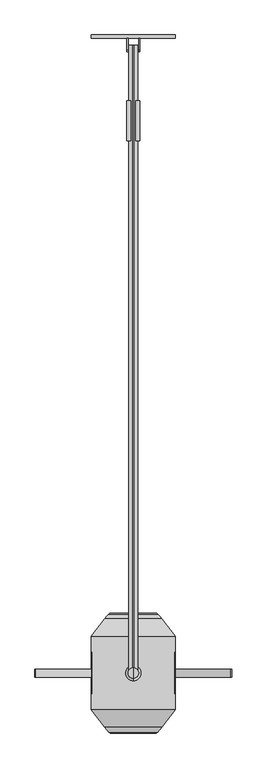
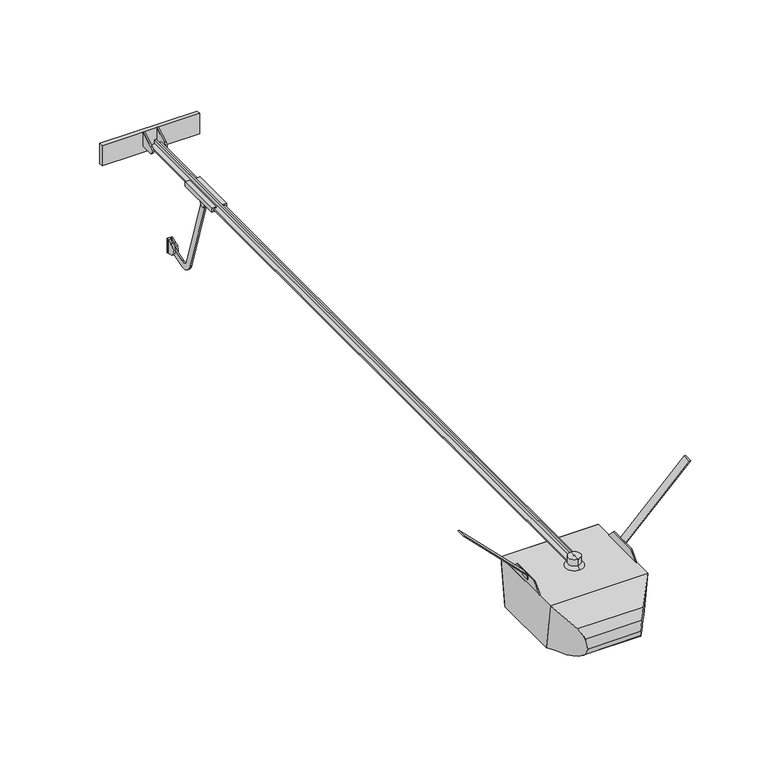
"""IFC4 building model written with IfcOpenShell, lengths in millimetres: proxy geometry, DoorOpener_Garage_Liftmaster_Residential-Standard : DoorOpener_Garage_Liftmaster_Residential-Standard."""

from ifc_helpers import new_model, si_unit, point, frame, frame_2d, origin, place, context, project, spatial, polyline, circle_curve, ellipse_curve, trimmed, segment, composite_curve, outline, extrude, source, transform, mapped, element, save
from ifc_brep_helpers import plane_surface, cylinder_surface, revolved_surface, advanced_brep


def specialty_equipment_f89a715d(model_context):
    return source(origin(), model_context, "Body", "SolidModel", [
        advanced_brep(
        [(-203.2, 149.6475517, -508.0003876), (203.2, 149.6475517, -508.0003876), (203.2, 177.8000484, -304.8), (-203.2, 177.8000484, -304.8), (138.0453476, 261.2609425, -380.4314301), (-138.0453476, 261.2609425, -380.4314301), (-118.4954842, 284.259248, -417.8810822), (118.4954842, 284.259248, -417.8810822), (-110.84057, 289.2573619, -461.4672022), (110.84057, 289.2573619, -461.4672022), (-116.7901976, 276.5450386, -491.3073174), (116.7901976, 276.5450386, -491.3073174), (-130.1422035, 255.1783195, -506.5798347), (130.1422035, 255.1783195, -506.5798347), (-170.8715769, 195.6710506, -512.2392761), (170.8715769, 195.6710506, -512.2392761)],
        [
            (0, 1),
            (1, 2),
            (2, 3),
            (3, 0),
            (2, 4, ellipse_curve(frame((725.3174618, -724.5630466, -1384.4430479), z_axis=(-0.8191520442889955, -0.5681495809146607, 0.0787145605568323), x_axis=(-0.5735764363510407, 0.8114016915146515, -0.11241604276082225)), 1717.7336421, 1407.0850245)),
            (4, 5),
            (5, 3, ellipse_curve(frame((-725.3174618, -724.5630466, -1384.4430479), z_axis=(0.8191520442889911, -0.5681495809146667, 0.07871456055683229), x_axis=(-0.573576436351047, -0.8114016915146469, 0.11241604276082202)), 1717.7336421, 1407.0850245)),
            (6, 5, ellipse_curve(frame((-176.0372598, 197.4858414, -445.3831284), z_axis=(0.8191520442889911, -0.5681495809146667, 0.07871456055683229), x_axis=(-0.573576436351047, -0.8114016915146469, 0.11241604276082202)), 111.1239307, 91.027395)),
            (4, 7, ellipse_curve(frame((176.0372598, 197.4858414, -445.3831284), z_axis=(-0.8191520442889955, -0.5681495809146607, 0.0787145605568323), x_axis=(-0.5735764363510407, 0.8114016915146515, -0.11241604276082225)), 111.1239307, 91.027395)),
            (7, 6),
            (8, 6, ellipse_curve(frame((-190.88231, 175.0994001, -452.4783085), z_axis=(0.8191520442889911, -0.5681495809146667, 0.07871456055683229), x_axis=(-0.573576436351047, -0.8114016915146469, 0.11241604276082202)), 139.7924992, 114.5113115)),
            (7, 9, ellipse_curve(frame((190.88231, 175.0994001, -452.4783085), z_axis=(-0.8191520442889955, -0.5681495809146607, 0.0787145605568323), x_axis=(-0.5735764363510407, 0.8114016915146515, -0.11241604276082225)), 139.7924992, 114.5113115)),
            (9, 8),
            (10, 8, ellipse_curve(frame((-146.4314203, 238.4966097, -457.470258), z_axis=(0.8191520442889911, -0.5681495809146667, 0.07871456055683229), x_axis=(-0.573576436351047, -0.8114016915146469, 0.11241604276082202)), 62.1592423, 50.9178704)),
            (9, 11, ellipse_curve(frame((146.4314203, 238.4966097, -457.470258), z_axis=(-0.8191520442889955, -0.5681495809146607, 0.0787145605568323), x_axis=(-0.5735764363510407, 0.8114016915146515, -0.11241604276082225)), 62.1592423, 50.9178704)),
            (11, 10),
            (12, 10, ellipse_curve(frame((-151.3050469, 232.2406655, -451.9067495), z_axis=(0.8191520442889911, -0.5681495809146667, 0.07871456055683229), x_axis=(-0.573576436351047, -0.8114016915146469, 0.11241604276082202)), 72.3795001, 59.2898155)),
            (11, 13, ellipse_curve(frame((151.3050469, 232.2406655, -451.9067495), z_axis=(-0.8191520442889955, -0.5681495809146607, 0.0787145605568323), x_axis=(-0.5735764363510407, 0.8114016915146515, -0.11241604276082225)), 72.3795001, 59.2898155)),
            (13, 12),
            (14, 12, ellipse_curve(frame((-165.9618007, 216.3547308, -414.0418022), z_axis=(0.8191520442889911, -0.5681495809146667, 0.07871456055683229), x_axis=(-0.573576436351047, -0.8114016915146469, 0.11241604276082202)), 122.507382, 100.3521724)),
            (13, 15, ellipse_curve(frame((165.9618007, 216.3547308, -414.0418022), z_axis=(-0.8191520442889955, -0.5681495809146607, 0.0787145605568323), x_axis=(-0.5735764363510407, 0.8114016915146515, -0.11241604276082225)), 122.507382, 100.3521724)),
            (15, 14),
            (0, 14, ellipse_curve(frame((-180.6608006, 154.4314578, -708.0276372), z_axis=(-0.8191520442889911, 0.5681495809146667, -0.07871456055683229), x_axis=(0.573576436351047, 0.8114016915146469, -0.11241604276082202)), 244.2580098, 200.0844481)),
            (15, 1, ellipse_curve(frame((180.6608006, 154.4314578, -708.0276372), z_axis=(0.8191520442889955, 0.5681495809146607, -0.0787145605568323), x_axis=(0.5735764363510407, -0.8114016915146515, 0.11241604276082225)), 244.2580098, 200.0844481)),
        ],
        [
            plane_surface(frame((-203.2, 149.6475517, -508.0003876), z_axis=(0.0, -0.9905385662791439, 0.13723464837153254), x_axis=(1.0, 0.0, 0.0))),
            cylinder_surface(frame((203.2, -724.5630466, -1384.4430479), z_axis=(-1.0, 0.0, 0.0), x_axis=(0.0, 1.0, 0.0)), 1407.0850245),
            cylinder_surface(frame((203.2, 197.4858414, -445.3831284), z_axis=(-1.0, 0.0, 0.0), x_axis=(0.0, 1.0, 0.0)), 91.027395),
            cylinder_surface(frame((203.2, 175.0994001, -452.4783085), z_axis=(-1.0, 0.0, 0.0), x_axis=(0.0, 1.0, 0.0)), 114.5113115),
            cylinder_surface(frame((203.2, 238.4966097, -457.470258), z_axis=(-1.0, 0.0, 0.0), x_axis=(0.0, 1.0, 0.0)), 50.9178704),
            cylinder_surface(frame((203.2, 232.2406655, -451.9067495), z_axis=(-1.0, 0.0, 0.0), x_axis=(0.0, 1.0, 0.0)), 59.2898155),
            cylinder_surface(frame((203.2, 216.3547308, -414.0418022), z_axis=(-1.0, 0.0, 0.0), x_axis=(0.0, 1.0, 0.0)), 100.3521724),
            revolved_surface(polyline([(320.7614394112816, 354.5159059, -708.0276372), (-320.7614394112831, 354.5159059, -708.0276372)]), (203.2, 154.4314578, -708.0276372), (1.0, 0.0, 0.0)),
            plane_surface(frame((-74.2567818, 321.5979485, -608.7511868), z_axis=(-0.8191520442889911, 0.5681495809146667, -0.07871456055683229), x_axis=(0.0, 0.13723464837153243, 0.9905385662791438))),
            plane_surface(frame((74.2567818, 369.5271494, -262.8055925), z_axis=(0.8191520442889955, 0.5681495809146607, -0.0787145605568323), x_axis=(0.0, -0.1372346483715328, -0.9905385662791438))),
        ],
        [
            (0, [[1, 2, 3, 4]]),
            (1, [[-3, 5, 6, 7]]),
            (2, [[8, -6, 9, 10]]),
            (3, [[11, -10, 12, 13]]),
            (4, [[14, -13, 15, 16]]),
            (5, [[17, -16, 18, 19]]),
            (6, [[20, -19, 21, 22]]),
            (7, [[-1, 23, -22, 24]]),
            (8, [[-4, -7, -8, -11, -14, -17, -20, -23]]),
            (9, [[-2, -24, -21, -18, -15, -12, -9, -5]]),
        ],
    ),
        extrude(outline(polyline([(177.8000484, -304.8), (149.6475517, -508.0003876), (-149.6475517, -508.0003876), (-177.8000484, -304.8), (177.8000484, -304.8)])), frame((-203.2, 0.0, 0.0), z_axis=(1.0, 0.0, 0.0), x_axis=(0.0, 1.0, 0.0)), (0.0, 0.0, 1.0), 406.4),
        advanced_brep(
        [(-203.2, -149.6475517, -508.0003876), (203.2, -149.6475517, -508.0003876), (170.8715769, -195.6710506, -512.2392761), (-170.8715769, -195.6710506, -512.2392761), (-130.1422035, -255.1783195, -506.5798347), (130.1422035, -255.1783195, -506.5798347), (-116.7901976, -276.5450386, -491.3073174), (116.7901976, -276.5450386, -491.3073174), (-110.84057, -289.2573619, -461.4672022), (110.84057, -289.2573619, -461.4672022), (-118.4954842, -284.259248, -417.8810822), (118.4954842, -284.259248, -417.8810822), (-138.0453476, -261.2609425, -380.4314301), (138.0453476, -261.2609425, -380.4314301), (203.2, -177.8000484, -304.8), (-203.2, -177.8000484, -304.8)],
        [
            (0, 1),
            (1, 2, ellipse_curve(frame((180.6608006, -154.4314578, -708.0276372), z_axis=(0.8191520442889902, -0.568149580914668, -0.07871456055683303), x_axis=(0.5735764363510483, 0.8114016915146459, 0.11241604276082269)), 244.2580098, 200.0844481)),
            (2, 3),
            (3, 0, ellipse_curve(frame((-180.6608006, -154.4314578, -708.0276372), z_axis=(-0.8191520442889942, -0.5681495809146623, -0.07871456055683314), x_axis=(0.5735764363510426, -0.8114016915146501, -0.11241604276082295)), 244.2580098, 200.0844481)),
            (4, 3, ellipse_curve(frame((-165.9618007, -216.3547308, -414.0418022), z_axis=(0.8191520442889942, 0.5681495809146623, 0.07871456055683314), x_axis=(-0.5735764363510426, 0.8114016915146501, 0.11241604276082295)), 122.507382, 100.3521724)),
            (2, 5, ellipse_curve(frame((165.9618007, -216.3547308, -414.0418022), z_axis=(-0.8191520442889902, 0.568149580914668, 0.07871456055683303), x_axis=(-0.5735764363510483, -0.8114016915146459, -0.11241604276082269)), 122.507382, 100.3521724)),
            (5, 4),
            (6, 4, ellipse_curve(frame((-151.3050469, -232.2406655, -451.9067495), z_axis=(0.8191520442889942, 0.5681495809146623, 0.07871456055683314), x_axis=(-0.5735764363510426, 0.8114016915146501, 0.11241604276082295)), 72.3795001, 59.2898155)),
            (5, 7, ellipse_curve(frame((151.3050469, -232.2406655, -451.9067495), z_axis=(-0.8191520442889902, 0.568149580914668, 0.07871456055683303), x_axis=(-0.5735764363510483, -0.8114016915146459, -0.11241604276082269)), 72.3795001, 59.2898155)),
            (7, 6),
            (8, 6, ellipse_curve(frame((-146.4314203, -238.4966097, -457.470258), z_axis=(0.8191520442889942, 0.5681495809146623, 0.07871456055683314), x_axis=(-0.5735764363510426, 0.8114016915146501, 0.11241604276082295)), 62.1592423, 50.9178704)),
            (7, 9, ellipse_curve(frame((146.4314203, -238.4966097, -457.470258), z_axis=(-0.8191520442889902, 0.568149580914668, 0.07871456055683303), x_axis=(-0.5735764363510483, -0.8114016915146459, -0.11241604276082269)), 62.1592423, 50.9178704)),
            (9, 8),
            (10, 8, ellipse_curve(frame((-190.88231, -175.0994001, -452.4783085), z_axis=(0.8191520442889942, 0.5681495809146623, 0.07871456055683314), x_axis=(-0.5735764363510426, 0.8114016915146501, 0.11241604276082295)), 139.7924992, 114.5113115)),
            (9, 11, ellipse_curve(frame((190.88231, -175.0994001, -452.4783085), z_axis=(-0.8191520442889902, 0.568149580914668, 0.07871456055683303), x_axis=(-0.5735764363510483, -0.8114016915146459, -0.11241604276082269)), 139.7924992, 114.5113115)),
            (11, 10),
            (12, 10, ellipse_curve(frame((-176.0372598, -197.4858414, -445.3831284), z_axis=(0.8191520442889942, 0.5681495809146623, 0.07871456055683314), x_axis=(-0.5735764363510426, 0.8114016915146501, 0.11241604276082295)), 111.1239307, 91.027395)),
            (11, 13, ellipse_curve(frame((176.0372598, -197.4858414, -445.3831284), z_axis=(-0.8191520442889902, 0.568149580914668, 0.07871456055683303), x_axis=(-0.5735764363510483, -0.8114016915146459, -0.11241604276082269)), 111.1239307, 91.027395)),
            (13, 12),
            (14, 15),
            (15, 12, ellipse_curve(frame((-725.3174618, 724.5630466, -1384.4430479), z_axis=(0.8191520442889942, 0.5681495809146623, 0.07871456055683314), x_axis=(-0.5735764363510426, 0.8114016915146501, 0.11241604276082295)), 1717.7336421, 1407.0850245)),
            (13, 14, ellipse_curve(frame((725.3174618, 724.5630466, -1384.4430479), z_axis=(-0.8191520442889902, 0.568149580914668, 0.07871456055683303), x_axis=(-0.5735764363510483, -0.8114016915146459, -0.11241604276082269)), 1717.7336421, 1407.0850245)),
            (0, 15),
            (14, 1),
        ],
        [
            revolved_surface(polyline([(320.7614394112834, -354.5159059, -708.0276372), (-320.76143941128197, -354.5159059, -708.0276372)]), (203.2, -154.4314578, -708.0276372), (1.0, 0.0, 0.0)),
            cylinder_surface(frame((203.2, -216.3547308, -414.0418022), z_axis=(-1.0, 0.0, 0.0), x_axis=(0.0, -1.0, 0.0)), 100.3521724),
            cylinder_surface(frame((203.2, -232.2406655, -451.9067495), z_axis=(-1.0, 0.0, 0.0), x_axis=(0.0, -1.0, 0.0)), 59.2898155),
            cylinder_surface(frame((203.2, -238.4966097, -457.470258), z_axis=(-1.0, 0.0, 0.0), x_axis=(0.0, -1.0, 0.0)), 50.9178704),
            cylinder_surface(frame((203.2, -175.0994001, -452.4783085), z_axis=(-1.0, 0.0, 0.0), x_axis=(0.0, -1.0, 0.0)), 114.5113115),
            cylinder_surface(frame((203.2, -197.4858414, -445.3831284), z_axis=(-1.0, 0.0, 0.0), x_axis=(0.0, -1.0, 0.0)), 91.027395),
            cylinder_surface(frame((203.2, 724.5630466, -1384.4430479), z_axis=(-1.0, 0.0, 0.0), x_axis=(0.0, -1.0, 0.0)), 1407.0850245),
            plane_surface(frame((-203.2, -177.8000484, -304.8), z_axis=(0.0, 0.9905385662791436, 0.13723464837153496), x_axis=(1.0, 0.0, 0.0))),
            plane_surface(frame((-203.2, -142.6760316, -558.3197467), z_axis=(-0.8191520442889942, -0.5681495809146623, -0.07871456055683314), x_axis=(0.0, -0.13723464837153365, 0.9905385662791437))),
            plane_surface(frame((203.2, -196.7053127, -168.3447132), z_axis=(0.81915204428899, -0.5681495809146679, -0.07871456055683301), x_axis=(0.0, 0.13723464837153368, -0.9905385662791437))),
        ],
        [
            (0, [[1, 2, 3, 4]]),
            (1, [[5, -3, 6, 7]]),
            (2, [[8, -7, 9, 10]]),
            (3, [[11, -10, 12, 13]]),
            (4, [[14, -13, 15, 16]]),
            (5, [[17, -16, 18, 19]]),
            (6, [[20, 21, -19, 22]]),
            (7, [[-1, 23, -20, 24]]),
            (8, [[-4, -5, -8, -11, -14, -17, -21, -23]]),
            (9, [[-2, -24, -22, -18, -15, -12, -9, -6]]),
        ],
    ),
        extrude(outline(polyline([(-285.75, -203.2), (-266.7, -203.2), (0.0, -469.9), (0.0, -474.3901281), (-268.0151281, -206.375), (-285.75, -206.375), (-285.75, -203.2)])), frame((0.0, -19.05, 0.0), z_axis=(0.0, 1.0, 0.0), x_axis=(0.0, 0.0, 1.0)), (0.0, 0.0, 1.0), 38.1),
        extrude(outline(polyline([(-285.75, 203.2), (-285.75, 206.375), (-268.0151281, 206.375), (0.0, 474.3901281), (0.0, 469.9), (-266.7, 203.2), (-285.75, 203.2)])), frame((0.0, -19.05, 0.0), z_axis=(0.0, 1.0, 0.0), x_axis=(0.0, 0.0, 1.0)), (0.0, 0.0, 1.0), 38.1),
        advanced_brep(
        [(31.75, 2758.489219, -277.7618368), (31.75, 2566.8381944, -277.7618368), (31.75, 2566.8381944, -296.0931426), (31.75, 2758.489219, -296.0931426), (-31.75, 2758.489219, -296.0931426), (-31.75, 2566.8381944, -296.0931426), (-31.75, 2566.8381944, -277.7618368), (-31.75, 2758.489219, -277.7618368), (9.525, 2758.489219, -296.0931426), (9.525, 2758.489219, -304.8), (-9.525, 2758.489219, -304.8), (-9.525, 2758.489219, -296.0931426), (-12.7, 2758.489219, -277.7618368), (-12.7, 2758.489219, -282.575), (-22.225, 2758.489219, -282.575), (-22.225, 2758.489219, -288.925), (22.225, 2758.489219, -288.925), (22.225, 2758.489219, -282.575), (12.7, 2758.489219, -282.575), (12.7, 2758.489219, -277.7618368), (12.7, 2566.8381944, -277.7618368), (-12.7, 2566.8381944, -277.7618368), (12.7, 2566.8381944, -282.575), (22.225, 2566.8381944, -282.575), (22.225, 2566.8381944, -288.925), (-22.225, 2566.8381944, -288.925), (-22.225, 2566.8381944, -282.575), (-12.7, 2566.8381944, -282.575), (-9.525, 2611.2881944, -296.0931426), (9.525, 2611.2881944, -296.0931426), (-9.525, 2616.3151009, -304.8), (9.525, 2616.3151009, -304.8), (-9.525, 2647.8709399, -304.8), (9.525, 2647.8709399, -304.8), (-9.525, 2658.7300795, -334.6352407), (9.525, 2658.7300795, -334.6352407), (-9.525, 2684.1300795, -334.6352407), (9.525, 2684.1300795, -334.6352407), (-9.525, 2694.989219, -304.8), (9.525, 2694.989219, -304.8)],
        [
            (0, 1),
            (1, 2),
            (2, 3),
            (3, 0),
            (4, 5),
            (5, 6),
            (6, 7),
            (7, 4),
            (3, 8),
            (8, 9),
            (9, 10),
            (10, 11),
            (11, 4),
            (7, 12),
            (12, 13),
            (13, 14),
            (14, 15),
            (15, 16),
            (16, 17),
            (17, 18),
            (18, 19),
            (19, 0),
            (19, 20),
            (20, 1),
            (6, 21),
            (21, 12),
            (5, 2),
            (20, 22),
            (22, 23),
            (23, 24),
            (24, 25),
            (25, 26),
            (26, 27),
            (27, 21),
            (11, 28),
            (28, 29),
            (29, 8),
            (28, 30),
            (30, 31),
            (31, 29),
            (30, 32),
            (32, 33),
            (33, 31),
            (32, 34),
            (34, 35),
            (35, 33),
            (34, 36, circle_curve(frame((-9.525, 2671.4300795, -330.0128187), z_axis=(1.0, 0.0, 0.0), x_axis=(0.0, 1.0, 0.0)), 13.5150577)),
            (36, 37),
            (37, 35, circle_curve(frame((9.525, 2671.4300795, -330.0128187), z_axis=(-1.0, 0.0, 0.0), x_axis=(0.0, 1.0, 0.0)), 13.5150577)),
            (36, 38),
            (38, 39),
            (39, 37),
            (9, 39),
            (38, 10),
            (13, 27),
            (26, 14),
            (25, 15),
            (24, 16),
            (23, 17),
            (22, 18),
        ],
        [
            plane_surface(frame((31.75, 2758.489219, -277.7618368), z_axis=(1.0, 0.0, 0.0), x_axis=(0.0, 0.0, 1.0))),
            plane_surface(frame((-31.75, 2758.489219, -277.7618368), z_axis=(-1.0, 0.0, 0.0), x_axis=(0.0, 0.0, -1.0))),
            plane_surface(frame((31.75, 2758.489219, -304.8), z_axis=(0.0, 1.0, 0.0), x_axis=(-1.0, 0.0, 0.0))),
            plane_surface(frame((31.75, 2758.489219, -277.7618368), z_axis=(0.0, 0.0, 1.0), x_axis=(-1.0, 0.0, 0.0))),
            plane_surface(frame((31.75, 2566.8381944, -277.7618368), z_axis=(0.0, -1.0, 0.0), x_axis=(-1.0, 0.0, 0.0))),
            plane_surface(frame((31.75, 2566.8381944, -296.0931426), z_axis=(0.0, 0.0, -1.0), x_axis=(-1.0, 0.0, 0.0))),
            plane_surface(frame((31.75, 2611.2881944, -296.0931426), z_axis=(0.0, -0.8660254037844414, -0.4999999999999954), x_axis=(-1.0, 0.0, 0.0))),
            plane_surface(frame((31.75, 2616.3151009, -304.8), z_axis=(0.0, 0.0, -1.0), x_axis=(-1.0, 0.0, 0.0))),
            plane_surface(frame((31.75, 2647.8709399, -304.8), z_axis=(0.0, -0.9396926207858758, -0.3420201433257583), x_axis=(-1.0, 0.0, 0.0))),
            cylinder_surface(frame((-31.75, 2671.4300795, -330.0128187), z_axis=(1.0, 0.0, 0.0), x_axis=(0.0, 1.0, 0.0)), 13.5150577),
            plane_surface(frame((31.75, 2684.1300795, -334.6352407), z_axis=(0.0, 0.939692620785905, -0.34202014332567826), x_axis=(-1.0, 0.0, 0.0))),
            plane_surface(frame((31.75, 2694.989219, -304.8), z_axis=(0.0, 0.0, -1.0), x_axis=(-1.0, 0.0, 0.0))),
            plane_surface(frame((-12.7, 2529.0462818, -282.575), z_axis=(0.0, 0.0, -1.0), x_axis=(0.0, 1.0, 0.0))),
            plane_surface(frame((-22.225, 2529.0462818, -282.575), z_axis=(1.0, 0.0, 0.0), x_axis=(0.0, 1.0, 0.0))),
            plane_surface(frame((-22.225, 2529.0462818, -288.925), z_axis=(0.0, 0.0, 1.0), x_axis=(0.0, 1.0, 0.0))),
            plane_surface(frame((22.225, 2529.0462818, -288.925), z_axis=(-1.0, 0.0, 0.0), x_axis=(0.0, 1.0, 0.0))),
            plane_surface(frame((22.225, 2529.0462818, -282.575), z_axis=(0.0, 0.0, -1.0), x_axis=(0.0, 1.0, 0.0))),
            plane_surface(frame((12.7, 2529.0462818, -282.575), z_axis=(-1.0, 0.0, 0.0), x_axis=(0.0, 1.0, 0.0))),
            plane_surface(frame((9.525, 2529.0462818, -296.0931426), z_axis=(1.0, 0.0, 0.0), x_axis=(0.0, 1.0, 0.0))),
            plane_surface(frame((-9.525, 2529.0462818, -350.5128419), z_axis=(-1.0, 0.0, 0.0), x_axis=(0.0, 1.0, 0.0))),
            plane_surface(frame((-12.7, 2529.0462818, -274.6526549), z_axis=(1.0, 0.0, 0.0), x_axis=(0.0, 1.0, 0.0))),
        ],
        [
            (0, [[1, 2, 3, 4]]),
            (1, [[5, 6, 7, 8]]),
            (2, [[-4, 9, 10, 11, 12, 13, -8, 14, 15, 16, 17, 18, 19, 20, 21, 22]]),
            (3, [[-1, -22, 23, 24]]),
            (3, [[-7, 25, 26, -14]]),
            (4, [[27, -2, -24, 28, 29, 30, 31, 32, 33, 34, -25, -6]]),
            (5, [[-13, 35, 36, 37, -9, -3, -27, -5]]),
            (6, [[-36, 38, 39, 40]]),
            (7, [[-39, 41, 42, 43]]),
            (8, [[-42, 44, 45, 46]]),
            (9, [[-45, 47, 48, 49]]),
            (10, [[-48, 50, 51, 52]]),
            (11, [[-11, 53, -51, 54]]),
            (12, [[55, -33, 56, -16]]),
            (13, [[-56, -32, 57, -17]]),
            (14, [[-57, -31, 58, -18]]),
            (15, [[-58, -30, 59, -19]]),
            (16, [[-59, -29, 60, -20]]),
            (17, [[-60, -28, -23, -21]]),
            (18, [[-37, -40, -43, -46, -49, -52, -53, -10]]),
            (19, [[-35, -12, -54, -50, -47, -44, -41, -38]]),
            (20, [[-55, -15, -26, -34]]),
        ],
    ),
        advanced_brep(
        [(0.0, 25.4, -263.525), (0.0, -25.4, -263.525), (0.0, 0.0, -263.525), (0.0, 25.4, -292.1), (0.0, -25.4, -292.1), (0.0, 38.1, -304.8), (0.0, -38.1, -304.8), (0.0, 0.0, -304.8)],
        [
            (0, 1, circle_curve(frame((0.0, 0.0, -263.525), z_axis=(0.0, 0.0, 1.0), x_axis=(0.0, -1.0, 0.0)), 25.4)),
            (1, 2),
            (2, 0),
            (1, 0, circle_curve(frame((0.0, 0.0, -263.525), z_axis=(0.0, 0.0, 1.0), x_axis=(0.0, -1.0, 0.0)), 25.4)),
            (3, 4, circle_curve(frame((0.0, 0.0, -292.1), z_axis=(0.0, 0.0, 1.0), x_axis=(0.0, -1.0, 0.0)), 25.4)),
            (4, 1),
            (0, 3),
            (4, 3, circle_curve(frame((0.0, 0.0, -292.1), z_axis=(0.0, 0.0, 1.0), x_axis=(0.0, -1.0, 0.0)), 25.4)),
            (5, 6, circle_curve(frame((0.0, 0.0, -304.8), z_axis=(0.0, 0.0, 1.0), x_axis=(0.0, -1.0, 0.0)), 38.1)),
            (6, 4),
            (3, 5),
            (6, 5, circle_curve(frame((0.0, 0.0, -304.8), z_axis=(0.0, 0.0, 1.0), x_axis=(0.0, -1.0, 0.0)), 38.1)),
            (7, 6),
            (5, 7),
        ],
        [
            plane_surface(frame((0.0, 0.0, -263.525), z_axis=(0.0, 0.0, 1.0), x_axis=(0.0, -1.0, 0.0))),
            cylinder_surface(frame((0.0, 0.0, -248.8162134), z_axis=(0.0, 0.0, -1.0), x_axis=(0.0, -1.0, 0.0)), 25.4),
            revolved_surface(polyline([(0.0, -25.4, -292.1), (0.0, -38.1, -304.8)]), (0.0, 0.0, -248.8162134), (0.0, 0.0, -1.0)),
            plane_surface(frame((0.0, 0.0, -304.8), z_axis=(0.0, 0.0, -1.0), x_axis=(0.0, -1.0, 0.0))),
        ],
        [
            (0, [[1, 2, 3]]),
            (0, [[4, -3, -2]]),
            (1, [[5, 6, -1, 7]]),
            (1, [[8, -7, -4, -6]]),
            (2, [[9, 10, -5, 11]]),
            (2, [[12, -11, -8, -10]]),
            (3, [[13, -9, 14]]),
            (3, [[-14, -12, -13]]),
        ],
    ),
        extrude(outline(polyline([(2924.175, -635.0), (2924.175, -698.5), (2917.825, -696.7985226), (2917.825, -636.7014774), (2924.175, -635.0)])), frame((-9.525, 0.0, 0.0), z_axis=(1.0, 0.0, 0.0), x_axis=(0.0, 1.0, 0.0)), (0.0, 0.0, 1.0), 19.05),
        extrude(outline(composite_curve([segment(polyline([(2924.175, -635.0), (2924.175, -698.5), (2897.2464471, -691.284516)]), True, "CONTINUOUS"), segment(trimmed(circle_curve(frame_2d((2903.8204508, -666.75)), 25.4), [point((2897.2464471, -691.284516))], [point((2897.2464471, -642.215484))], False, "CARTESIAN"), True, "CONTINUOUS"), segment(polyline([(2897.2464471, -642.215484), (2924.175, -635.0)]), True, "CONTINUOUS")], self_intersect=False)), frame((-9.525, 0.0, 0.0), z_axis=(1.0, 0.0, 0.0), x_axis=(0.0, 1.0, 0.0)), (0.0, 0.0, 1.0), 6.35),
        extrude(outline(composite_curve([segment(trimmed(circle_curve(frame_2d((2903.8204508, -666.75)), 12.7), [point((2899.895935, -654.6715822))], [point((2907.7449666, -678.8284178))], False, "CARTESIAN"), True, "CONTINUOUS"), segment(polyline([(2907.7449666, -678.8284178), (2835.2744601, -702.3755127)]), True, "CONTINUOUS"), segment(trimmed(circle_curve(frame_2d((2819.5763968, -654.0618417)), 50.8), [point((2835.2744601, -702.3755127))], [point((2771.2627258, -669.759905))], False, "CARTESIAN"), True, "CONTINUOUS"), segment(polyline([(2771.2627258, -669.759905), (2651.564993, -301.3681634), (2675.7218285, -293.5191318), (2795.4195613, -661.9108734)]), True, "CONTINUOUS"), segment(trimmed(circle_curve(frame_2d((2819.5763968, -654.0618417)), 25.4), [point((2795.4195613, -661.9108734))], [point((2827.4254284, -678.2186772))], True, "CARTESIAN"), True, "CONTINUOUS"), segment(polyline([(2827.4254284, -678.2186772), (2899.895935, -654.6715822)]), True, "CONTINUOUS")], self_intersect=False)), frame((-3.175, 0.0, 0.0), z_axis=(1.0, 0.0, 0.0), x_axis=(0.0, 1.0, 0.0)), (0.0, 0.0, 1.0), 6.35),
        extrude(outline(composite_curve([segment(polyline([(2924.175, -635.0), (2924.175, -698.5), (2897.2464471, -691.284516)]), True, "CONTINUOUS"), segment(trimmed(circle_curve(frame_2d((2903.8204508, -666.75)), 25.4), [point((2897.2464471, -691.284516))], [point((2897.2464471, -642.215484))], False, "CARTESIAN"), True, "CONTINUOUS"), segment(polyline([(2897.2464471, -642.215484), (2924.175, -635.0)]), True, "CONTINUOUS")], self_intersect=False)), frame((3.175, 0.0, 0.0), z_axis=(1.0, 0.0, 0.0), x_axis=(0.0, 1.0, 0.0)), (0.0, 0.0, 1.0), 6.35),
        extrude(outline(polyline([(-282.575, -3.175), (-282.575, -22.225), (-288.925, -22.225), (-288.925, 22.225), (-282.575, 22.225), (-282.575, 3.175), (-263.525, 3.175), (-263.525, -3.175), (-282.575, -3.175)])), frame((0.0, 0.0, 0.0), z_axis=(0.0, 1.0, 0.0), x_axis=(0.0, 0.0, 1.0)), (0.0, 0.0, 1.0), 3025.775),
        extrude(outline(composite_curve([segment(polyline([(3060.7, -304.8), (3005.7074265, -304.8)]), True, "CONTINUOUS"), segment(trimmed(circle_curve(frame_2d((3014.8728406, -288.925)), 18.3308604), [point((3005.7074265, -304.8))], [point((3005.7074265, -273.05))], False, "CARTESIAN"), True, "CONTINUOUS"), segment(polyline([(3005.7074265, -273.05), (3060.7, -241.3000969), (3060.7, -304.8)]), True, "CONTINUOUS")], self_intersect=False)), frame((-31.75, 0.0, 0.0), z_axis=(1.0, 0.0, 0.0), x_axis=(0.0, 1.0, 0.0)), (0.0, 0.0, 1.0), 6.35),
        extrude(outline(composite_curve([segment(polyline([(3060.7, -304.8), (3005.7074265, -304.8)]), True, "CONTINUOUS"), segment(trimmed(circle_curve(frame_2d((3014.8728406, -288.925)), 18.3308604), [point((3005.7074265, -304.8))], [point((3005.7074265, -273.05))], False, "CARTESIAN"), True, "CONTINUOUS"), segment(polyline([(3005.7074265, -273.05), (3060.7, -241.3000969), (3060.7, -304.8)]), True, "CONTINUOUS")], self_intersect=False)), frame((25.4, 0.0, 0.0), z_axis=(1.0, 0.0, 0.0), x_axis=(0.0, 1.0, 0.0)), (0.0, 0.0, 1.0), 6.35),
        extrude(outline(polyline([(-203.2, 3076.575), (203.2, 3076.575), (203.2, 3060.7), (-203.2, 3060.7), (-203.2, 3076.575)])), frame((0.0, 0.0, -330.2), z_axis=(0.0, 0.0, 1.0), x_axis=(1.0, 0.0, 0.0)), (0.0, 0.0, 1.0), 88.8999031),
        extrude(outline(polyline([(-101.5999031, -304.8), (-63.4999031, -266.7), (63.5000484, -266.7), (101.6000484, -304.8), (-101.5999031, -304.8)])), frame((200.025, 0.0, 0.0), z_axis=(1.0, 0.0, 0.0), x_axis=(0.0, 1.0, 0.0)), (0.0, 0.0, 1.0), 3.175),
        extrude(outline(polyline([(-101.5999031, -304.8), (-63.4999031, -266.7), (63.5000484, -266.7), (101.6000484, -304.8), (-101.5999031, -304.8)])), frame((-203.2, 0.0, 0.0), z_axis=(1.0, 0.0, 0.0), x_axis=(0.0, 1.0, 0.0)), (0.0, 0.0, 1.0), 3.175),
    ])


if __name__ == "__main__":
    model = new_model("IFC4")
    model_context = context("Model", 3, world=origin())
    ifc_project = project(units=[si_unit("LENGTHUNIT", "METRE", prefix="MILLI")], contexts=[model_context])
    site = spatial("IfcSite", under=ifc_project)
    building = spatial("IfcBuilding", under=site)
    placement = place(None, origin())
    specialty_equipment_shape = specialty_equipment_f89a715d(model_context)
    element("IfcBuildingElementProxy", 1, Name="DoorOpener_Garage_Liftmaster_Residential-Standard : DoorOpener_Garage_Liftmaster_Residential-Standard", ObjectType="DoorOpener_Garage_Liftmaster_Residential-Standard : DoorOpener_Garage_Liftmaster_Residential-Standard", at=placement, inside=building, context=model_context, shape_type="MappedRepresentation", body=[
        mapped(specialty_equipment_shape, transform((0.0, 0.0, 0.0), x_axis=(1.0, 0.0, 0.0), y_axis=(0.0, 1.0, 0.0), z_axis=(0.0, 0.0, 1.0))),
    ])
    save(model, "model.ifc")

# Revit data of these elements
# Type "DoorOpener_Garage_Liftmaster_Residential-Standard : DoorOpener_Garage_Liftmaster_Residential-Standard"
#   COBie.Type.CreatedBy = "info@geappliances.com"
#   COBie.Type.CreatedOn = "2017-07-20T03:49:29"
#   COBie.Type.Name = "DoorOpener_Garage_Liftmaster_Residential-Standard_DoorOpener_Garage_Liftmaster_Residential-Standard"
#   COBie.Type.Category = "E1030900"
#   COBie.Type.Description = "DoorOpener_Garage_Liftmaster_Residential-Standard_DoorOpener_Garage_Liftmaster_Residential-Standard"
#   COBie.Type.Manufacturer = "specs@liftmaster.com"
#   COBie.Type.ModelNumber = "As Specified"
#   URL = "http://www.liftmaster.com/consumerweb"
#   Specification = "http://www.arcat.com/sd/clients/chamber.html?coid=42485"
#   SpecWizard = ""
#   Send Message = "http://www.arcat.com/users.pl?action=UserEmail&company=LiftMaster%20-%20The%20Chamberlain%20Group,%20Inc.%20%20&coid=42485&rep=111&fax=877-361-9589&mf="
#   Sales Information = "http://www.liftmaster.com/consumerweb/service"
#   Revision = "R1_07-2011"
#   Product Properties = ""
#   Product Data = "http://www.arcat.com/arcatcos/cos42/arc42485.html"
#   Model = "As Specified"
#   Manufacturer Website = "http://www.liftmaster.com/consumerweb"
#   Manufacturer Phone - Toll Free = "800-282-6225 "
#   Manufacturer Phone = ""
#   Manufacturer Fax = "877-361-9589"
#   Manufacturer Address = "845 Larch Ave. Elmhurst, IL 60126"
#   Manufacturer = "specs@liftmaster.com"
#   Keynote = "08730"
#   Installation-Fabrication = "http://www.liftmaster.com/consumerweb/service/manuals"
#   Installation Phase = ""
#   Green Building-LEED = "http://www.arcat.com/green/clients/leed_data_42485.html"
#   Drive Type = ""
#   Drawn By = "Sumex Design, Inc. / Robert S. Weygant, CSI, CDT, SCIP"
#   Description = "LiftMaster"
#   Copyright = "©Arcat Inc."
#   Construction Details = "http://www.arcat.com/details/chamber/chamber.html?coid=42485"
#   Assembly Code = "E1030900"
#   COBie.Type.ReplacementCost = 0
#   offset [instance default] = 0' - 0"
#   Unit Width = 1' - 4"
#   Unit Height = 0' - 8 1/4"
#   Unit Depth = 1' - 10 7/8"
#   Track Length [instance default] = 10' - 0"
#   Support Strap Angle [instance default] = 45.00°
#   Support Connection Extension [instance default] = 0' - 6"
#   Sup Offset [instance default] = 0' - 0"
#   Mounting Drop [instance default] = 1' - 0"
#   Motor HP = 0
#   Max Door Height = 0' - 0"
#   Width [instance default] = 1' - 4"
#   Head Rotation [instance default] = 90.00°
#   Depth [instance default] = 1' - 10 7/8"
#   Default Elevation = 4' - 0"
#   COBie.Type = yes
#   Warranty Duration (Years) = 0
#   Rotated Motor Mounting [instance default] = no
#   Maintenance Schedule (Months) = 0
#   Has Battery Backup = no
#   Expected Lifespan (Years) = 0
#   Cover = no
#   2nd Light Compartment = yes
#   Track Material = Metal - Aluminum - Liftmaster - Anodized - Clear
#   Support Material = Metal - Steel - Liftmaster - Powder Coat - Black
#   Material = Plastic - Liftmaster - Red
#   Accent Material = Plastic - Liftmaster - White
# Element 1 (IfcBuildingElementProxy, "DoorOpener_Garage_Liftmaster_Residential-Standard : DoorOpener_Garage_Liftmaster_Residential-Standard")
#   Track Length = 9' - 7 1/8"
#   Materials on its faces: "Metal - Steel - Liftmaster - Powder Coat - Black", "Plastic - Liftmaster - White", "Metal - Aluminum - Liftmaster - Anodized - Clear", "Plastic - Liftmaster - Red"
# Materials
#   "Metal - Aluminum - Liftmaster - Anodized - Clear": class "Metal", colour RGB 237 237 237, transparency 0, Comments = "Anodized Aluminum - Clear", Description = "Anodized Aluminum - Clear", Cost = 0
#   "Metal - Steel - Liftmaster - Powder Coat - Black": class "Metal", colour RGB 17 17 17, transparency 0, Comments = "Powder Coat Steel - Black", Description = "Powder Coat Steel - Black", Cost = 0
#   "Plastic - Liftmaster - Red": class "Plastic", colour RGB 140 0 0, transparency 0, Comments = "Plastic - Red", Description = "Plastic - Red", Cost = 0
#   "Plastic - Liftmaster - White": class "Plastic", colour RGB 234 234 234, transparency 0, Comments = "Plastic - White", Description = "Plastic - White", Cost = 0
